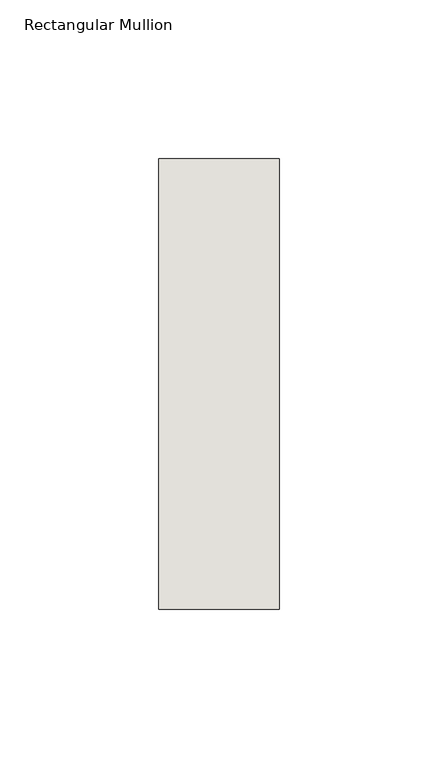
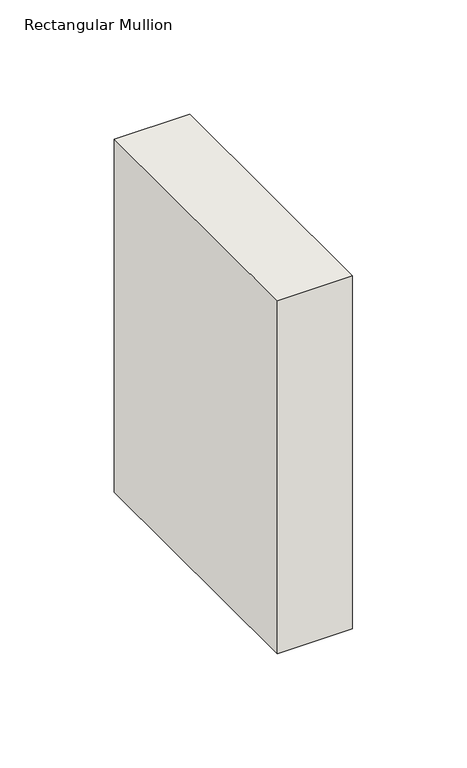
"""IFC4 building model written with IfcOpenShell, lengths in millimetres: wall geometry, Rectangular Mullion : NLRS_21_CWM_hsb-regel 38x142_gen_rsf."""

from ifc_helpers import new_model, si_unit, frame, origin, place, context, project, spatial, polyline, outline, extrude, source, transform, mapped, element, save


def rectangular_mullion_db279188(model_context):
    return source(origin(), model_context, "Body", "SweptSolid", [
        extrude(outline(polyline([(-38.0, -71.0), (-38.0, 71.0), (0.0, 71.0), (0.0, -71.0), (-38.0, -71.0)])), frame((0.0, 0.0, -187.9999997), z_axis=(0.0, 0.0, 1.0), x_axis=(1.0, 0.0, 0.0)), (0.0, 0.0, 1.0), 187.9999997),
    ])


if __name__ == "__main__":
    model = new_model("IFC4")
    model_context = context("Model", 3, world=origin())
    ifc_project = project(units=[si_unit("LENGTHUNIT", "METRE", prefix="MILLI")], contexts=[model_context])
    site = spatial("IfcSite", under=ifc_project)
    building = spatial("IfcBuilding", under=site)
    placement = place(None, origin())
    rectangular_mullion_shape = rectangular_mullion_db279188(model_context)
    element("IfcWall", 1, ObjectType="Rectangular Mullion : NLRS_21_CWM_hsb-regel 38x142_gen_rsf", at=placement, inside=building, context=model_context, shape_type="MappedRepresentation", body=[
        mapped(rectangular_mullion_shape, transform((0.0, 0.0, 0.0), x_axis=(1.0, 0.0, 0.0), y_axis=(0.0, 1.0, 0.0), z_axis=(0.0, 0.0, 1.0))),
    ])
    save(model, "model.ifc")

# Revit data of these elements
# Type "Rectangular Mullion : NLRS_21_CWM_hsb-regel 38x142_gen_rsf"
#   Type IfcGUID = "07M7mRoiH1CR8m_RSKIwpF"
#   Assembly Code = "21.10"
#   IfcExportAs = "IfcWall"
#   built-in parameter 1007322 = 0.465879 (stored number, unit not read)
#   built-in parameter 1007321 = 0.062336 (stored number, unit not read)
#   built-in parameter 1007320 = 0.062336 (stored number, unit not read)
# Element 1 (IfcWall, "Rectangular Mullion : NLRS_21_CWM_hsb-regel 38x142_gen_rsf")
#   Materials on its faces: "NLRS_i2_hout naaldhout vuren_gen_rsf"
# Materials
#   "NLRS_i2_hout naaldhout vuren_gen_rsf": class "I - Hout", colour RGB 234 199 147, transparency 0, Keynote = "i2", Manufacturer = "Revit Standards Foundation", URL = "www.revitstandards.org", Description = "hout vuren", Cost = 0
